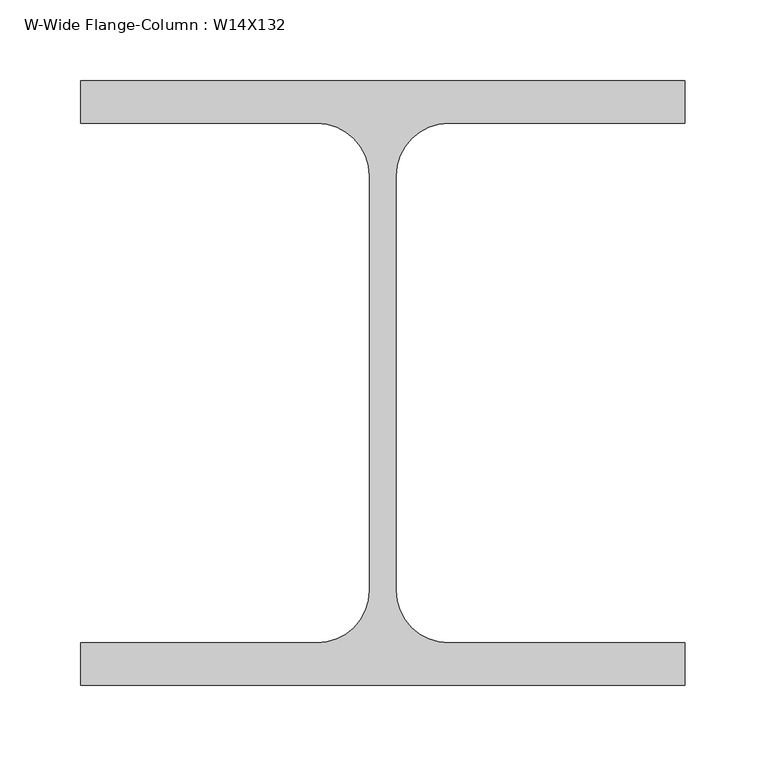
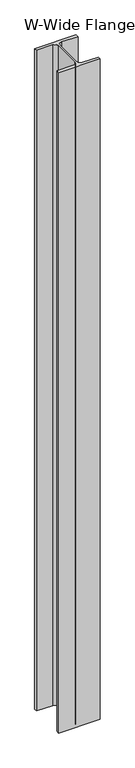
"""IFC4 building model written with IfcOpenShell, lengths in millimetres: column geometry, W-Wide Flange-Column : W14X132."""

from ifc_helpers import new_model, si_unit, point, frame, frame_2d, origin, place, context, project, spatial, polyline, circle_curve, trimmed, segment, composite_curve, outline, extrude, source, transform, mapped, element, save


def w_wide_flange_column_w14x132_1d26bb89(model_context):
    return source(origin(), model_context, "Body", "SweptSolid", [
        extrude(outline(composite_curve([segment(polyline([(186.69, -186.69), (-186.69, -186.69), (-186.69, -160.528), (-40.767, -160.528)]), True, "CONTINUOUS"), segment(trimmed(circle_curve(frame_2d((-40.767, -127.9525)), 32.5755), [point((-40.767, -160.528))], [point((-8.1915, -127.9525))], True, "CARTESIAN"), True, "CONTINUOUS"), segment(polyline([(-8.1915, -127.9525), (-8.1915, 127.9525)]), True, "CONTINUOUS"), segment(trimmed(circle_curve(frame_2d((-40.767, 127.9525)), 32.5755), [point((-8.1915, 127.9525))], [point((-40.767, 160.528))], True, "CARTESIAN"), True, "CONTINUOUS"), segment(polyline([(-40.767, 160.528), (-186.69, 160.528), (-186.69, 186.69), (186.69, 186.69), (186.69, 160.528), (40.767, 160.528)]), True, "CONTINUOUS"), segment(trimmed(circle_curve(frame_2d((40.767, 127.9525)), 32.5755), [point((40.767, 160.528))], [point((8.1915, 127.9525))], True, "CARTESIAN"), True, "CONTINUOUS"), segment(polyline([(8.1915, 127.9525), (8.1915, -127.9525)]), True, "CONTINUOUS"), segment(trimmed(circle_curve(frame_2d((40.767, -127.9525)), 32.5755), [point((8.1915, -127.9525))], [point((40.767, -160.528))], True, "CARTESIAN"), True, "CONTINUOUS"), segment(polyline([(40.767, -160.528), (186.69, -160.528), (186.69, -186.69)]), True, "CONTINUOUS")], self_intersect=False)), frame((0.0, 0.0, -304.8), z_axis=(0.0, 0.0, 1.0), x_axis=(1.0, 0.0, 0.0)), (0.0, 0.0, 1.0), 6273.8),
    ])


if __name__ == "__main__":
    model = new_model("IFC4")
    model_context = context("Model", 3, world=origin())
    ifc_project = project(units=[si_unit("LENGTHUNIT", "METRE", prefix="MILLI")], contexts=[model_context])
    site = spatial("IfcSite", under=ifc_project)
    building = spatial("IfcBuilding", under=site)
    placement = place(None, origin())
    w_wide_flange_column_w14x132_shape = w_wide_flange_column_w14x132_1d26bb89(model_context)
    element("IfcColumn", 1, ObjectType="W-Wide Flange-Column : W14X132", at=placement, inside=building, context=model_context, shape_type="MappedRepresentation", body=[
        mapped(w_wide_flange_column_w14x132_shape, transform((0.0, 0.0, 0.0), x_axis=(1.0, 0.0, 0.0), y_axis=(0.0, 1.0, 0.0), z_axis=(0.0, 0.0, 1.0))),
    ])
    save(model, "model.ifc")

# Revit data of these elements
# Type "W-Wide Flange-Column : W14X132"
#   Assembly Code = "B10"
#   W = 132
#   bf = 1' - 2.7"
#   d = 1' - 2.7"
#   k = 0' - 2 5/16"
#   kr = 0' - 1.2825"
#   tf = 0' - 1.03"
#   tw = 0' - 0.645"
#   A = 0.269444 SF
#   Column Material [instance default] = Metal - Steel - ASTM A992
# Element 1 (IfcColumn, "W-Wide Flange-Column : W14X132")
#   Materials on its faces: "Metal - Steel - ASTM A992"
# Materials
#   "Metal - Steel - ASTM A992": class "Metal", colour RGB 128 0 0, transparency 0
